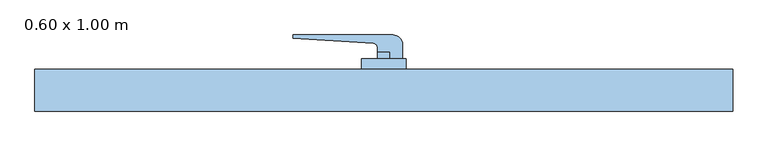
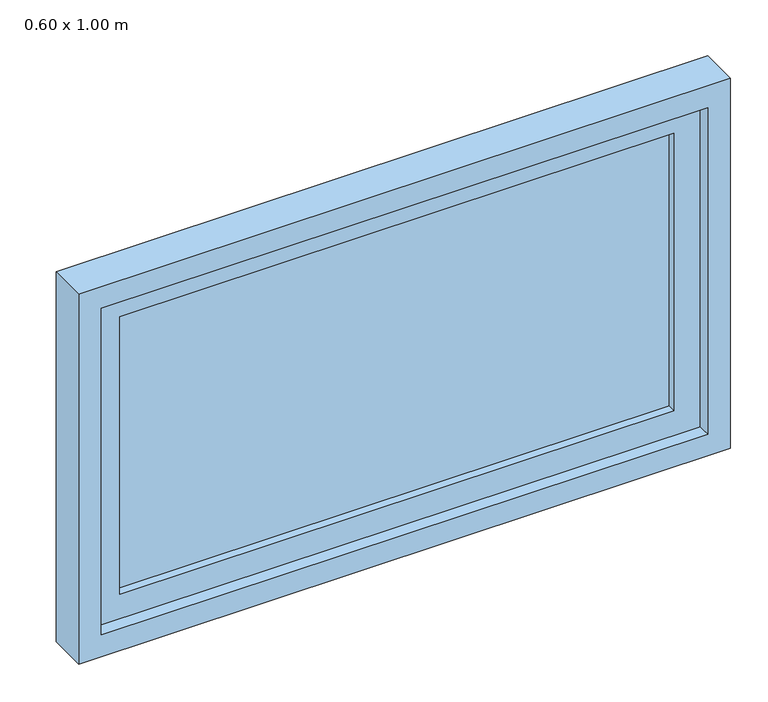
"""IFC4 building model written with IfcOpenShell, lengths in millimetres: window geometry, Janela maxim-ar - 1 Painel : 0.60 x 1.00 m."""

from ifc_helpers import new_model, si_unit, point, frame, frame_2d, origin, place, context, project, spatial, polyline, circle_curve, trimmed, segment, composite_curve, outline, extrude, source, transform, mapped, element, save


def window_0_60_x_1_00_m_96a756a1(model_context):
    return source(origin(), model_context, "Body", "SweptSolid", [
        extrude(outline(composite_curve([segment(polyline([(9.0, 110.0), (-9.0, 110.0), (-9.0, 115.9630874)]), True, "CONTINUOUS"), segment(trimmed(circle_curve(frame_2d((-15.0369126, 115.9630874)), 6.0369126), [point((-9.0, 115.9630874))], [point((-14.6705919, 121.9888756))], True, "CARTESIAN"), True, "CONTINUOUS"), segment(polyline([(-14.6705919, 121.9888756), (-130.0, 129.0), (-130.0, 134.0), (13.0, 134.0)]), True, "CONTINUOUS"), segment(trimmed(circle_curve(frame_2d((13.0, 120.0)), 14.0), [point((13.0, 134.0))], [point((27.0, 120.0))], False, "CARTESIAN"), True, "CONTINUOUS"), segment(polyline([(27.0, 120.0), (27.0, 100.0), (9.0, 100.0), (9.0, 110.0)]), True, "CONTINUOUS")], self_intersect=False)), frame((0.0, 0.0, 707.0), z_axis=(0.0, 0.0, 1.0), x_axis=(1.0, 0.0, 0.0)), (0.0, 0.0, 1.0), 16.0),
        extrude(outline(polyline([(723.0, 9.0), (723.0, -9.0), (703.0135985, -9.0), (685.0, -6.9842809), (685.0, 7.0348924), (703.0135985, 9.0), (723.0, 9.0)])), frame((0.0, 100.0, 0.0), z_axis=(0.0, 1.0, 0.0), x_axis=(0.0, 0.0, 1.0)), (0.0, 0.0, 1.0), 10.0),
        extrude(outline(polyline([(32.0, 100.0), (32.0, 85.0), (-32.0, 85.0), (-32.0, 100.0), (32.0, 100.0)])), frame((0.0, 0.0, 705.0), z_axis=(0.0, 0.0, 1.0), x_axis=(1.0, 0.0, 0.0)), (0.0, 0.0, 1.0), 20.0),
        extrude(outline(polyline([(425.0, 58.0), (-425.0, 58.0), (-425.0, 72.0), (425.0, 72.0), (425.0, 58.0)])), frame((0.0, 0.0, 725.0), z_axis=(0.0, 0.0, 1.0), x_axis=(1.0, 0.0, 0.0)), (0.0, 0.0, 1.0), 450.0),
        extrude(outline(polyline([(1215.0, -465.0), (685.0, -465.0), (685.0, 465.0), (1215.0, 465.0), (1215.0, -465.0)]), holes=[polyline([(725.0, -425.0), (1175.0, -425.0), (1175.0, 425.0), (725.0, 425.0), (725.0, -425.0)])]), frame((0.0, 45.0, 0.0), z_axis=(0.0, 1.0, 0.0), x_axis=(0.0, 0.0, 1.0)), (0.0, 0.0, 1.0), 40.0),
        extrude(outline(polyline([(1250.0, -500.0), (650.0, -500.0), (650.0, 500.0), (1250.0, 500.0), (1250.0, -500.0)]), holes=[polyline([(685.0, -465.0), (1215.0, -465.0), (1215.0, 465.0), (685.0, 465.0), (685.0, -465.0)])]), frame((0.0, 25.0, 0.0), z_axis=(0.0, 1.0, 0.0), x_axis=(0.0, 0.0, 1.0)), (0.0, 0.0, 1.0), 60.0),
    ])


if __name__ == "__main__":
    model = new_model("IFC4")
    model_context = context("Model", 3, world=origin())
    ifc_project = project(units=[si_unit("LENGTHUNIT", "METRE", prefix="MILLI")], contexts=[model_context])
    site = spatial("IfcSite", under=ifc_project)
    building = spatial("IfcBuilding", under=site)
    placement = place(None, origin())
    window_0_60_x_1_00_m_shape = window_0_60_x_1_00_m_96a756a1(model_context)
    element("IfcWindow", 1, ObjectType="Janela maxim-ar - 1 Painel : 0.60 x 1.00 m", at=placement, inside=building, context=model_context, shape_type="MappedRepresentation", body=[
        mapped(window_0_60_x_1_00_m_shape, transform((0.0, 0.0, 0.0), x_axis=(1.0, 0.0, 0.0), y_axis=(0.0, 1.0, 0.0), z_axis=(0.0, 0.0, 1.0))),
    ])
    save(model, "model.ifc")

# Revit data of these elements
# Type "Janela maxim-ar - 1 Painel : 0.60 x 1.00 m"
#   Type Mark = "J21"
#   Construction Type Id = "SGL"
#   Analytic Construction = "Janelas grandes envidraçadas únicas"
#   Visual Light Transmittance = 0.9
#   Solar Heat Gain Coefficient = 0.86
#   Rough Width = 1.000 m
#   Rough Height = 0.600 m
#   Largura da moldura do painel = 0.040 m
#   Espessura da moldura do painel = 0.040 m
#   Height = 0.600 m
#   Heat Transfer Coefficient (U) = 5.5617 W/(m²·K)
#   Largura da estrutura = 0.035 m
#   Espessura da moldura = 0.060 m
#   Altura-padrão do peitoril = 0.650 m
#   Width = 1.000 m
#   Material do puxador = Metal - Alumínio
#   Vidro = Vidro
#   Material da estrutura = Metal - Alumínio
#   Wall Closure = (empty or 0)
# Element 1 (IfcWindow, "Janela maxim-ar - 1 Painel : 0.60 x 1.00 m")
#   Materials on its faces: "Metal - Alumínio", "Vidro"
# Materials
#   "Metal - Alumínio": class "Metal", colour RGB 247 247 247, transparency 0
#   "Vidro": class "Vidro", colour RGB 0 128 192, transparency 0.9
